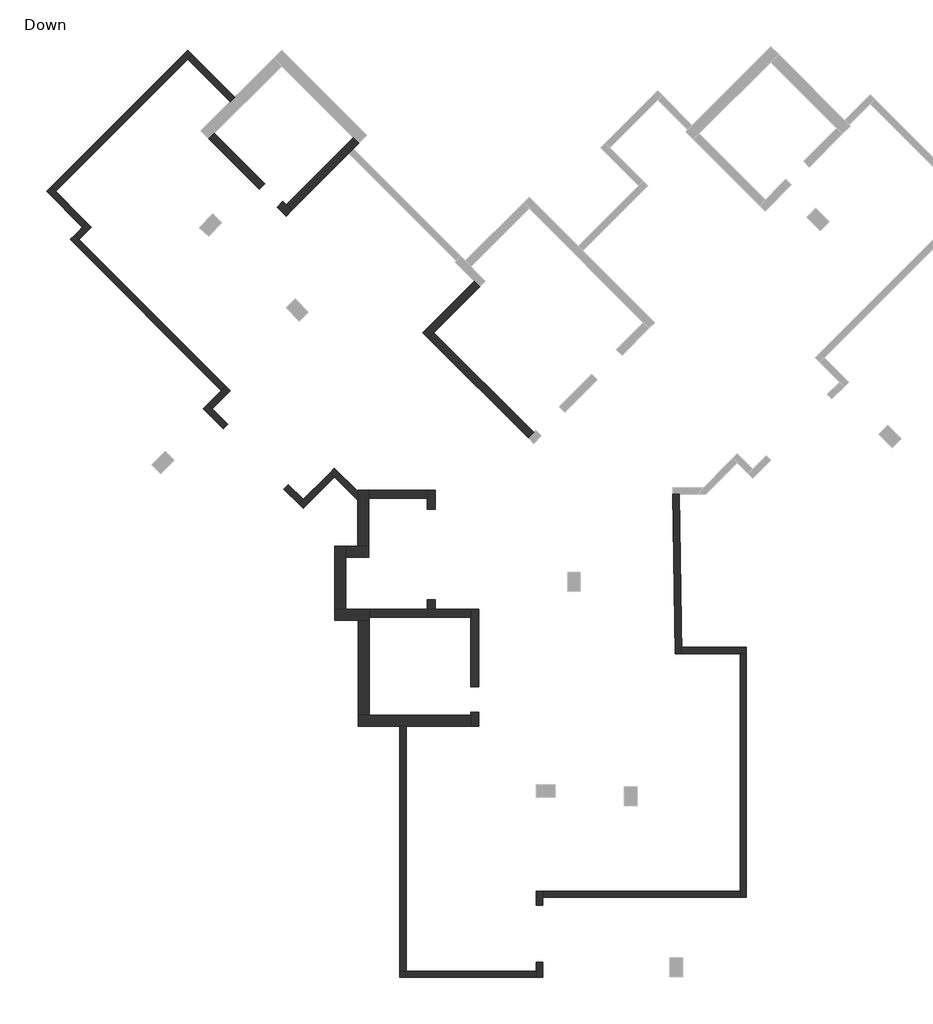
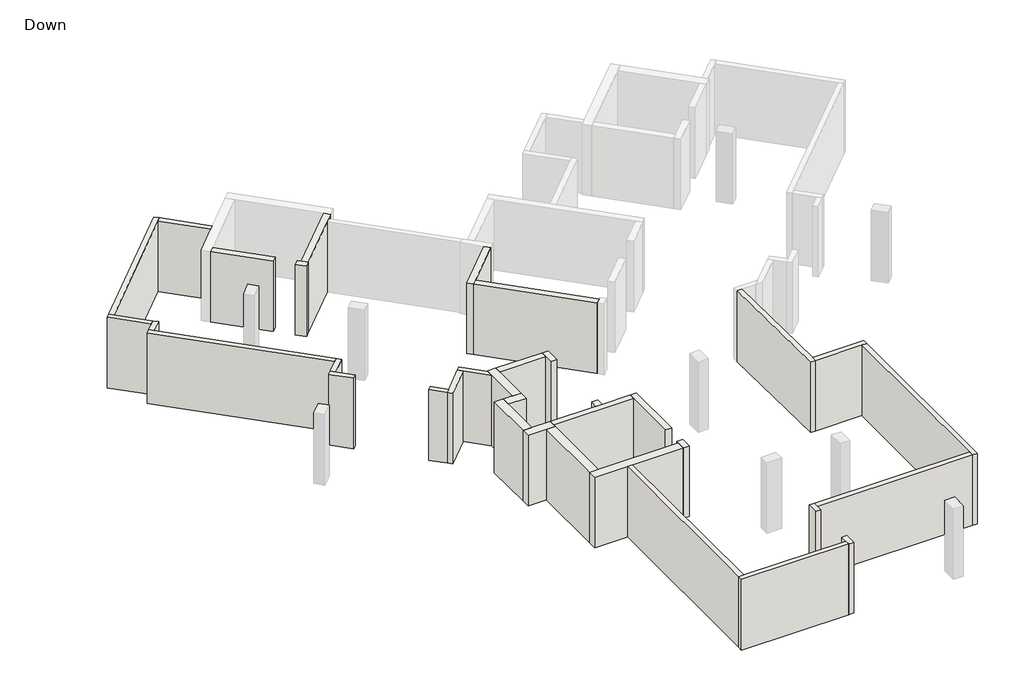
# One storey, part 1 of 2: 35 walls.
"""IFC4 building model written with IfcOpenShell, lengths in millimetres."""

import ifcopenshell
import ifcopenshell.guid

model = None  # the IFC model being written
_history = None  # IfcOwnerHistory: only IFC2X3 demands one
_inside = {}  # id of a spatial element -> (the spatial element, [elements in it])
_under = {}  # id of a project, library or spatial element -> (it, [spatial elements below it])
_declared = {}  # id of a project -> (the project, [libraries it declares])
_typed = {}  # id of a type object -> (the type object, [elements of that type])
_made_of = {}  # id of a material, layer set ... -> (it, [elements and type objects made of it])


def new_model(schema):
    """Start an empty IFC model of exactly this schema.

    Asked for "IFC4X3", IfcOpenShell would pick the latest addendum, in which some entities
    have other attributes; the version numbers below select the first issue.
    IFC2X3 requires an IfcOwnerHistory on every rooted entity: one is made here for all.
    """
    global model, _history
    if schema == "IFC4X3":
        model = ifcopenshell.file(schema_version=(4, 3, 0, 0))
    else:
        model = ifcopenshell.file(schema=schema)
    _inside.clear()
    _under.clear()
    _declared.clear()
    _typed.clear()
    _made_of.clear()
    _history = None
    if model.schema == "IFC2X3":
        org = make("IfcOrganization", Name="unknown")
        user = make(
            "IfcPersonAndOrganization",
            ThePerson=make("IfcPerson", FamilyName="unknown"),
            TheOrganization=org,
        )
        app = make(
            "IfcApplication",
            ApplicationDeveloper=org,
            Version="unknown",
            ApplicationFullName="unknown",
            ApplicationIdentifier="unknown",
        )
        _history = make(
            "IfcOwnerHistory",
            OwningUser=user,
            OwningApplication=app,
            ChangeAction="ADDED",
            CreationDate=0,
        )
    return model


def make(cls, **values):
    """One entity of the class cls with the attributes given. An attribute that is None is left unset."""
    return model.create_entity(
        cls, **{name: value for name, value in values.items() if value is not None}
    )


def rooted(cls, **values):
    """An entity with a GlobalId (a new one), such as an element, a storey or a relation."""
    return make(cls, GlobalId=ifcopenshell.guid.new(), OwnerHistory=_history, **values)


def si_unit(unit_type, name, prefix=None):
    """IfcSIUnit, for example si_unit("LENGTHUNIT", "METRE", prefix="MILLI")."""
    return make("IfcSIUnit", UnitType=unit_type, Prefix=prefix, Name=name)


def assignment(units):
    """IfcUnitAssignment: the units of a project."""
    return None if units is None else make("IfcUnitAssignment", Units=units)


def point(xyz):
    """IfcCartesianPoint."""
    return None if xyz is None else make("IfcCartesianPoint", Coordinates=xyz)


def direction(xyz):
    """IfcDirection."""
    return None if xyz is None else make("IfcDirection", DirectionRatios=xyz)


def frame(location, z_axis=None, x_axis=None):
    """IfcAxis2Placement3D, a coordinate frame: its origin and axes. An axis left out is left unset."""
    return make(
        "IfcAxis2Placement3D",
        Location=point(location),
        Axis=direction(z_axis),
        RefDirection=direction(x_axis),
    )


def origin():
    """The frame at (0, 0, 0) with its axes left unset."""
    return frame((0.0, 0.0, 0.0))


def origin_with_axes():
    """The frame at (0, 0, 0) with the z axis (0, 0, 1) and the x axis (1, 0, 0) written out."""
    return frame((0.0, 0.0, 0.0), z_axis=(0.0, 0.0, 1.0), x_axis=(1.0, 0.0, 0.0))


def place(relative_to, where):
    """IfcLocalPlacement: puts the frame where relative to a parent placement (None: the world)."""
    return make(
        "IfcLocalPlacement", PlacementRelTo=relative_to, RelativePlacement=where
    )


def context(
    kind, dimensions, precision=None, world=None, true_north=None, identifier=None
):
    """IfcGeometricRepresentationContext, for example the 3D "Model" context."""
    return make(
        "IfcGeometricRepresentationContext",
        ContextIdentifier=identifier,
        ContextType=kind,
        CoordinateSpaceDimension=dimensions,
        Precision=precision,
        WorldCoordinateSystem=world,
        TrueNorth=true_north,
    )


def project(units=None, contexts=None):
    """IfcProject with its units and contexts."""
    return rooted(
        "IfcProject",
        Name="project",
        RepresentationContexts=contexts,
        UnitsInContext=assignment(units),
    )


def spatial(cls, under=None, at=None, **own):
    """A site, building, storey or space (cls), placed at a placement, below another one or the project."""
    s = rooted(cls, ObjectPlacement=at, **own)
    if under is not None:
        _under.setdefault(under.id(), (under, []))[1].append(s)
    return s


def polyline(points):
    """IfcPolyline through the points."""
    return make("IfcPolyline", Points=[point(p) for p in points])


def outline(outer, holes=None, kind="AREA"):
    """IfcArbitraryClosedProfileDef: a profile drawn as a closed curve; with holes, ...WithVoids."""
    if holes is None:
        return make("IfcArbitraryClosedProfileDef", ProfileType=kind, OuterCurve=outer)
    return make(
        "IfcArbitraryProfileDefWithVoids",
        ProfileType=kind,
        OuterCurve=outer,
        InnerCurves=holes,
    )


def extrude(swept, where, along, depth):
    """IfcExtrudedAreaSolid: the profile swept, set in the frame where, extruded along a direction by depth."""
    return make(
        "IfcExtrudedAreaSolid",
        SweptArea=swept,
        Position=where,
        ExtrudedDirection=direction(along),
        Depth=depth,
    )


def faces_of(points, faces, orient=None, outer=None):
    """IfcFace entities. A face is a list of loops; a loop is a list of indices into points, from 0.

    orient and outer hold one flag for each loop. By default every Orientation is true, the
    first loop of a face is its IfcFaceOuterBound and the others are IfcFaceBound.
    """
    made = []
    for i, loops in enumerate(faces):
        bounds = []
        for j, loop in enumerate(loops):
            is_outer = j == 0 if outer is None else outer[i][j]
            bounds.append(
                make(
                    "IfcFaceOuterBound" if is_outer else "IfcFaceBound",
                    Bound=make("IfcPolyLoop", Polygon=[points[k] for k in loop]),
                    Orientation=True if orient is None else orient[i][j],
                )
            )
        made.append(make("IfcFace", Bounds=bounds))
    return made


def faceted_brep(points, faces, orient=None, outer=None, voids=None):
    """IfcFacetedBrep: a solid bounded by flat faces; with voids (closed shells), ...WithVoids."""
    shared = [point(p) for p in points]
    hull = make("IfcClosedShell", CfsFaces=faces_of(shared, faces, orient, outer))
    if voids is None:
        return make("IfcFacetedBrep", Outer=hull)
    return make(
        "IfcFacetedBrepWithVoids",
        Outer=hull,
        Voids=[
            make(cls, CfsFaces=faces_of(shared, fs, o, b)) for cls, fs, o, b in voids
        ],
    )


def shape(context_of_items, identifier, shape_type, items):
    """IfcShapeRepresentation: the items that make up one representation, for example the "Body"."""
    return make(
        "IfcShapeRepresentation",
        ContextOfItems=context_of_items,
        RepresentationIdentifier=identifier,
        RepresentationType=shape_type,
        Items=items,
    )


def made_of(thing, what):
    """Note that an element or type object is made of a material, layer set ...; save() writes the relation."""
    if what is not None:
        _made_of.setdefault(what.id(), (what, []))[1].append(thing)
    return thing


def element(
    cls,
    number,
    at=None,
    inside=None,
    cuts=None,
    type_object=None,
    material=None,
    context=None,
    identifier="Body",
    shape_type=None,
    held_by="IfcProductDefinitionShape",
    body=None,
    shapes=None,
    **own,
):
    """One element of the class cls, such as IfcWall. Its Tag is "e" and its number.

    at: its placement. inside: the storey or other place that contains it. cuts: it is an
    opening in that element (IfcRelVoidsElement). A single representation is given by context,
    identifier, shape_type and body (its items); several are given by shapes. held_by: the class
    of the entity that holds the representations. save() writes the other relations.
    """
    e = rooted(cls, Tag="e%d" % number, ObjectPlacement=at, **own)
    if body is not None:
        shapes = [shape(context, identifier, shape_type, body)]
    if shapes is not None:
        e.Representation = make(held_by, Representations=shapes)
    if inside is not None:
        _inside.setdefault(inside.id(), (inside, []))[1].append(e)
    if cuts is not None:
        rooted(
            "IfcRelVoidsElement", RelatingBuildingElement=cuts, RelatedOpeningElement=e
        )
    if type_object is not None:
        _typed.setdefault(type_object.id(), (type_object, []))[1].append(e)
    return made_of(e, material)


def aggregate(whole, parts):
    """IfcRelAggregates: a whole, such as a stair, and the parts it consists of."""
    return rooted("IfcRelAggregates", RelatingObject=whole, RelatedObjects=parts)


def save(model, path):
    """Write the relations noted so far, then the file.

    IfcRelAggregates (storeys below a building ...), IfcRelContainedInSpatialStructure (elements
    in a storey), IfcRelDefinesByType, IfcRelAssociatesMaterial and IfcRelDeclares: one each for
    every whole, place, type object, material and project.
    """
    for whole, parts in _under.values():
        aggregate(whole, parts)
    for where, things in _inside.values():
        rooted(
            "IfcRelContainedInSpatialStructure",
            RelatedElements=things,
            RelatingStructure=where,
        )
    for kind, things in _typed.values():
        rooted("IfcRelDefinesByType", RelatedObjects=things, RelatingType=kind)
    for what, things in _made_of.values():
        rooted("IfcRelAssociatesMaterial", RelatedObjects=things, RelatingMaterial=what)
    for by, libraries in _declared.values():
        rooted("IfcRelDeclares", RelatingContext=by, RelatedDefinitions=libraries)
    model.write(path)


model = new_model("IFC4")

# Units and contexts
model_context = context("Model", 3, world=origin())
ifc_project = project(units=[si_unit("LENGTHUNIT", "METRE", prefix="MILLI")], contexts=[model_context])

# Site, building, storey
site = spatial("IfcSite", under=ifc_project)
building = spatial("IfcBuilding", under=site)
storey = spatial("IfcBuildingStorey", under=building, Name="Down", Elevation=0.0)

# Walls
placement = place(None, origin())
element("IfcWall", 1, ObjectType="20", at=placement, inside=storey, context=model_context, shape_type="Brep", body=[
    faceted_brep([(-4151.5371537, 1666.662681, 0.0), (-4879.6277554, 2394.7532827, 0.0), (-4879.6277554, 2394.7532827, 2820.0), (-4879.6277554, 2394.7532827, 3000.0), (-4151.5371537, 1666.662681, 3000.0), (-4151.5371537, 1666.662681, 2820.0), (-4151.5371537, 1383.8199686, 0.0), (-4151.5371537, 1383.8199686, 3000.0), (-4879.6277554, 2111.9105702, 3000.0), (-5021.0491116, 2253.3319265, 3000.0), (-5021.0491116, 2253.3319265, 0.0), (-4879.6277554, 2111.9105702, 0.0)], [[[0, 1, 2, 3, 4, 5]], [[6, 7, 8, 9, 10, 11]], [[1, 0, 6, 11, 10]], [[4, 3, 9, 8, 7]], [[3, 2, 1, 10, 9]], [[0, 5, 4, 7, 6]]]),
])
element("IfcWall", 2, ObjectType="20", at=placement, inside=storey, context=model_context, shape_type="Brep", body=[
    faceted_brep([(-5021.0491116, 2253.3319265, 0.0), (-5869.5772491, 1404.803789, 0.0), (-6010.9986053, 1263.3824328, 0.0), (-6010.9986053, 1263.3824328, 3000.0), (-5869.5772491, 1404.803789, 3000.0), (-5021.0491116, 2253.3319265, 3000.0), (-4879.6277554, 2111.9105702, 0.0), (-4879.6277554, 2111.9105702, 3000.0), (-5869.5772491, 1121.9610766, 3000.0), (-5869.5772491, 1121.9610766, 0.0), (-5945.8975357, 1198.2813632, 3000.0)], [[[0, 1, 2, 3, 4, 5]], [[6, 7, 8, 9]], [[2, 1, 0, 6, 9]], [[5, 4, 3, 10, 8, 7]], [[0, 5, 7, 6]], [[3, 2, 9, 8, 10]]]),
])
element("IfcWall", 3, ObjectType="20", at=placement, inside=storey, context=model_context, shape_type="Brep", body=[
    faceted_brep([(-5869.5772491, 1404.803789, 0.0), (-6335.1870225, 1870.4135624, 0.0), (-6335.1870225, 1870.4135624, 2820.0), (-6335.1870225, 1870.4135624, 3000.0), (-5869.5772491, 1404.803789, 3000.0), (-5869.5772491, 1404.803789, 2820.0), (-6010.9986053, 1263.3824328, 0.0), (-6010.9986053, 1263.3824328, 3000.0), (-6476.6083787, 1728.9922062, 3000.0), (-6476.6083787, 1728.9922062, 2820.0), (-6476.6083787, 1728.9922062, 0.0)], [[[0, 1, 2, 3, 4, 5]], [[6, 7, 8, 9, 10]], [[1, 0, 6, 10]], [[3, 2, 1, 10, 9, 8]], [[4, 3, 8, 7]], [[0, 5, 4, 7, 6]]]),
])
element("IfcWall", 4, ObjectType="20", at=placement, inside=storey, context=model_context, shape_type="Brep", body=[
    faceted_brep([(-8243.933641, 3779.160181, 0.0), (-8738.7611577, 4273.9876976, 0.0), (-8880.1825139, 4415.4090539, 0.0), (-8880.1825139, 4415.4090539, 3000.0), (-8738.7611577, 4273.9876976, 3000.0), (-8243.933641, 3779.160181, 3000.0), (-8243.933641, 3779.160181, 2820.0), (-8385.3549973, 3637.7388248, 0.0), (-8385.3549973, 3637.7388248, 2820.0), (-8385.3549973, 3637.7388248, 3000.0), (-8946.5252944, 4198.9091219, 3000.0), (-9021.6038701, 4273.9876976, 3000.0), (-9021.6038701, 4273.9876976, 0.0)], [[[0, 1, 2, 3, 4, 5, 6]], [[7, 8, 9, 10, 11, 12]], [[2, 1, 0, 7, 12]], [[5, 4, 3, 11, 10, 9]], [[0, 6, 5, 9, 8, 7]], [[3, 2, 12, 11]]]),
])
element("IfcWall", 5, ObjectType="20", at=placement, inside=storey, context=model_context, shape_type="Brep", body=[
    faceted_brep([(-8738.7611577, 4273.9876976, 0.0), (-8172.2562086, 4840.4926467, 0.0), (-8172.2562086, 4840.4926467, 2820.0), (-8172.2562086, 4840.4926467, 3000.0), (-8738.7611577, 4273.9876976, 3000.0), (-8738.7611577, 4273.9876976, 2820.0), (-8880.1825139, 4415.4090539, 0.0), (-8880.1825139, 4415.4090539, 3000.0), (-8455.0989211, 4840.4926467, 3000.0), (-8313.6775649, 4981.9140029, 3000.0), (-8313.6775649, 4981.9140029, 0.0), (-8455.0989211, 4840.4926467, 0.0)], [[[0, 1, 2, 3, 4, 5]], [[6, 7, 8, 9, 10, 11]], [[1, 0, 6, 11, 10]], [[4, 3, 9, 8, 7]], [[0, 5, 4, 7, 6]], [[3, 2, 1, 10, 9]]]),
])
element("IfcWall", 6, ObjectType="20", at=placement, inside=storey, context=model_context, shape_type="Brep", body=[
    faceted_brep([(-8313.6775649, 4981.9140029, 0.0), (-12945.5654963, 9613.8019343, 0.0), (-13086.9868525, 9755.2232905, 0.0), (-13086.9868525, 9755.2232905, 3000.0), (-12945.5654963, 9613.8019343, 3000.0), (-8313.6775649, 4981.9140029, 3000.0), (-13228.4082088, 9613.8019343, 0.0), (-8455.0989211, 4840.4926467, 0.0), (-8455.0989211, 4840.4926467, 3000.0), (-13228.4082088, 9613.8019343, 3000.0)], [[[0, 1, 2, 3, 4, 5]], [[6, 7, 8, 9]], [[2, 1, 0, 7, 6]], [[5, 4, 3, 9, 8]], [[3, 2, 6, 9]], [[0, 5, 8, 7]]]),
])
element("IfcWall", 7, ObjectType="20", at=placement, inside=storey, context=model_context, shape_type="Brep", body=[
    faceted_brep([(-12945.5654963, 9613.8019343, 0.0), (-12556.7794585, 10002.5879721, 0.0), (-12556.7794585, 10002.5879721, 2820.0), (-12556.7794585, 10002.5879721, 3000.0), (-12945.5654963, 9613.8019343, 3000.0), (-12945.5654963, 9613.8019343, 2820.0), (-13086.9868525, 9755.2232905, 0.0), (-13086.9868525, 9755.2232905, 3000.0), (-12839.6221709, 10002.5879721, 3000.0), (-12698.2008147, 10144.0093284, 3000.0), (-12698.2008147, 10144.0093284, 0.0), (-12839.6221709, 10002.5879721, 0.0)], [[[0, 1, 2, 3, 4, 5]], [[6, 7, 8, 9, 10, 11]], [[1, 0, 6, 11, 10]], [[4, 3, 9, 8, 7]], [[0, 5, 4, 7, 6]], [[3, 2, 1, 10, 9]]]),
])
element("IfcWall", 8, ObjectType="20", at=placement, inside=storey, context=model_context, shape_type="Brep", body=[
    faceted_brep([(-12698.2008147, 10144.0093284, 0.0), (-13688.6426542, 11134.4511678, 0.0), (-13830.0640104, 11275.8725241, 0.0), (-13830.0640104, 11275.8725241, 3000.0), (-13688.6426542, 11134.4511678, 3000.0), (-12698.2008147, 10144.0093284, 3000.0), (-12839.6221709, 10002.5879721, 0.0), (-12839.6221709, 10002.5879721, 3000.0), (-13971.4853667, 11134.4511678, 3000.0), (-13971.4853667, 11134.4511678, 0.0)], [[[0, 1, 2, 3, 4, 5]], [[6, 7, 8, 9]], [[2, 1, 0, 6, 9]], [[5, 4, 3, 8, 7]], [[0, 5, 7, 6]], [[3, 2, 9, 8]]]),
])
element("IfcWall", 9, ObjectType="20", at=placement, inside=storey, context=model_context, shape_type="Brep", body=[
    faceted_brep([(-13688.6426542, 11134.4511678, 0.0), (-9516.9564504, 15306.1373716, 0.0), (-9375.5350942, 15447.5587279, 0.0), (-9375.5350942, 15447.5587279, 3000.0), (-9516.9564504, 15306.1373716, 3000.0), (-13688.6426542, 11134.4511678, 3000.0), (-13688.6426542, 11134.4511678, 2820.0), (-13830.0640104, 11275.8725241, 0.0), (-13830.0640104, 11275.8725241, 3000.0), (-9516.9564504, 15588.9800841, 3000.0), (-9516.9564504, 15588.9800841, 0.0)], [[[0, 1, 2, 3, 4, 5, 6]], [[7, 8, 9, 10]], [[2, 1, 0, 7, 10]], [[5, 4, 3, 9, 8]], [[0, 6, 5, 8, 7]], [[3, 2, 10, 9]]]),
])
element("IfcWall", 10, ObjectType="20", at=placement, inside=storey, context=model_context, shape_type="Brep", body=[
    faceted_brep([(-9516.9564504, 15306.1373716, 0.0), (-8173.4037002, 13962.5846214, 0.0), (-8173.4037002, 13962.5846214, 2820.0), (-8173.4037002, 13962.5846214, 3000.0), (-9516.9564504, 15306.1373716, 3000.0), (-9516.9564504, 15306.1373716, 2820.0), (-9375.5350942, 15447.5587279, 0.0), (-9375.5350942, 15447.5587279, 3000.0), (-8031.9823439, 14104.0059776, 3000.0), (-8031.9823439, 14104.0059776, 0.0)], [[[0, 1, 2, 3, 4, 5]], [[6, 7, 8, 9]], [[1, 0, 6, 9]], [[4, 3, 8, 7]], [[0, 5, 4, 7, 6]], [[3, 2, 1, 9, 8]]]),
])
element("IfcWall", 11, ObjectType="20", at=placement, inside=storey, context=model_context, shape_type="Brep", body=[
    faceted_brep([(5808.4890075, 1568.8966142, 0.0), (5879.1909347, -3458.8761541, 0.0), (5879.1909347, -3458.8761541, 2820.0), (5879.1909347, -3458.8761541, 3000.0), (5808.4890075, 1568.8966142, 3000.0), (6008.5087812, 1568.8966142, 0.0), (6008.5087812, 1568.8966142, 3000.0), (6076.3982534, -3258.8761541, 3000.0), (6079.2107085, -3458.8761541, 3000.0), (6079.2107085, -3458.8761541, 0.0), (6076.3982534, -3258.8761541, 0.0)], [[[0, 1, 2, 3, 4]], [[5, 6, 7, 8, 9, 10]], [[1, 0, 5, 10, 9]], [[4, 3, 8, 7, 6]], [[0, 4, 6, 5]], [[3, 2, 1, 9, 8]]]),
])
element("IfcWall", 12, ObjectType="20", at=placement, inside=storey, context=model_context, shape_type="Brep", body=[
    faceted_brep([(6079.2107085, -3458.8761541, 0.0), (7926.5061285, -3458.8761541, 0.0), (8126.5061285, -3458.8761541, 0.0), (8126.5061285, -3458.8761541, 3000.0), (7926.5061285, -3458.8761541, 3000.0), (6079.2107085, -3458.8761541, 3000.0), (6076.3982534, -3258.8761541, 0.0), (6076.3982534, -3258.8761541, 3000.0), (8126.5061285, -3258.8761541, 3000.0), (8126.5061285, -3258.8761541, 0.0)], [[[0, 1, 2, 3, 4, 5]], [[6, 7, 8, 9]], [[2, 1, 0, 6, 9]], [[5, 4, 3, 8, 7]], [[0, 5, 7, 6]], [[3, 2, 9, 8]]]),
])
element("IfcWall", 13, ObjectType="20", at=placement, inside=storey, context=model_context, shape_type="Brep", body=[
    faceted_brep([(7926.5061285, -3458.8761541, 0.0), (7926.5061285, -10958.0646121, 0.0), (7926.5061285, -11158.0646121, 0.0), (7926.5061285, -11158.0646121, 3000.0), (7926.5061285, -10958.0646121, 3000.0), (7926.5061285, -3458.8761541, 3000.0), (7926.5061285, -3458.8761541, 2820.0), (8126.5061285, -3458.8761541, 0.0), (8126.5061285, -3458.8761541, 3000.0), (8126.5061285, -11158.0646121, 3000.0), (8126.5061285, -11158.0646121, 0.0)], [[[0, 1, 2, 3, 4, 5, 6]], [[7, 8, 9, 10]], [[2, 1, 0, 7, 10]], [[5, 4, 3, 9, 8]], [[0, 6, 5, 8, 7]], [[3, 2, 10, 9]]]),
])
element("IfcWall", 14, ObjectType="20", at=placement, inside=storey, context=model_context, shape_type="Brep", body=[
    faceted_brep([(7926.5061285, -10958.0646121, 0.0), (1689.535885, -10958.0646121, 0.0), (1689.535885, -10958.0646121, 3000.0), (7926.5061285, -10958.0646121, 3000.0), (7926.5061285, -10958.0646121, 2820.0), (7926.5061285, -11158.0646121, 0.0), (7926.5061285, -11158.0646121, 3000.0), (6112.9804297, -11158.0646121, 3000.0), (1689.535885, -11158.0646121, 3000.0), (1689.535885, -11158.0646121, 2820.0), (1689.535885, -11158.0646121, 0.0)], [[[0, 1, 2, 3, 4]], [[5, 6, 7, 8, 9, 10]], [[1, 0, 5, 10]], [[3, 2, 8, 7, 6]], [[0, 4, 3, 6, 5]], [[2, 1, 10, 9, 8]]]),
])
element("IfcWall", 15, ObjectType="20", at=placement, inside=storey, context=model_context, shape_type="Brep", body=[
    faceted_brep([(1489.535885, -10958.0646121, 0.0), (1489.535885, -11409.1015824, 0.0), (1489.535885, -11409.1015824, 2820.0), (1489.535885, -11409.1015824, 3000.0), (1489.535885, -10958.0646121, 3000.0), (1489.535885, -10958.0646121, 2820.0), (1689.535885, -10958.0646121, 0.0), (1689.535885, -10958.0646121, 3000.0), (1689.535885, -11158.0646121, 3000.0), (1689.535885, -11409.1015824, 3000.0), (1689.535885, -11409.1015824, 2820.0), (1689.535885, -11409.1015824, 0.0), (1689.535885, -11158.0646121, 0.0)], [[[0, 1, 2, 3, 4, 5]], [[6, 7, 8, 9, 10, 11, 12]], [[1, 0, 6, 12, 11]], [[3, 2, 1, 11, 10, 9]], [[4, 3, 9, 8, 7]], [[0, 5, 4, 7, 6]]]),
])
element("IfcWall", 16, ObjectType="20", at=placement, inside=storey, context=model_context, shape_type="Brep", body=[
    faceted_brep([(1489.535885, -13208.1998691, 0.0), (1489.535885, -13487.1899503, 0.0), (1489.535885, -13687.1899503, 0.0), (1489.535885, -13687.1899503, 3000.0), (1489.535885, -13487.1899503, 3000.0), (1489.535885, -13208.1998691, 3000.0), (1489.535885, -13208.1998691, 2820.0), (1689.535885, -13208.1998691, 0.0), (1689.535885, -13208.1998691, 2820.0), (1689.535885, -13208.1998691, 3000.0), (1689.535885, -13687.1899503, 3000.0), (1689.535885, -13687.1899503, 2820.0), (1689.535885, -13687.1899503, 0.0), (1589.2653711, -13687.1899503, 3000.0)], [[[0, 1, 2, 3, 4, 5, 6]], [[7, 8, 9, 10, 11, 12]], [[2, 1, 0, 7, 12]], [[5, 4, 3, 13, 10, 9]], [[0, 6, 5, 9, 8, 7]], [[3, 2, 12, 11, 10, 13]]]),
])
element("IfcWall", 17, ObjectType="20", at=placement, inside=storey, context=model_context, shape_type="Brep", body=[
    faceted_brep([(1489.535885, -13487.1899503, 0.0), (-2615.4235379, -13487.1899503, 0.0), (-2815.4235379, -13487.1899503, 0.0), (-2815.4235379, -13487.1899503, 3000.0), (-2615.4235379, -13487.1899503, 3000.0), (1489.535885, -13487.1899503, 3000.0), (1489.535885, -13487.1899503, 2820.0), (1489.535885, -13687.1899503, 0.0), (1489.535885, -13687.1899503, 3000.0), (-2815.4235379, -13687.1899503, 3000.0), (-2815.4235379, -13687.1899503, 0.0)], [[[0, 1, 2, 3, 4, 5, 6]], [[7, 8, 9, 10]], [[2, 1, 0, 7, 10]], [[5, 4, 3, 9, 8]], [[0, 6, 5, 8, 7]], [[3, 2, 10, 9]]]),
])
element("IfcWall", 18, ObjectType="20", at=placement, inside=storey, context=model_context, shape_type="Brep", body=[
    faceted_brep([(-2615.4235379, -13487.1899503, 0.0), (-2615.4235379, -5759.3270107, 0.0), (-2615.4235379, -5759.3270107, 2820.0), (-2615.4235379, -5759.3270107, 3000.0), (-2615.4235379, -13487.1899503, 3000.0), (-2615.4235379, -13487.1899503, 2820.0), (-2815.4235379, -13487.1899503, 0.0), (-2815.4235379, -13487.1899503, 3000.0), (-2815.4235379, -5759.3270107, 3000.0), (-2815.4235379, -5759.3270107, 0.0)], [[[0, 1, 2, 3, 4, 5]], [[6, 7, 8, 9]], [[1, 0, 6, 9]], [[4, 3, 8, 7]], [[0, 5, 4, 7, 6]], [[3, 2, 1, 9, 8]]]),
])
element("IfcWall", 19, ObjectType="25", at=placement, inside=storey, context=model_context, shape_type="Brep", body=[
    faceted_brep([(-8848.1886442, 12792.8249306, 0.0), (-7257.2630329, 11201.8993193, 0.0), (-7257.2630329, 11201.8993193, 2820.0), (-7257.2630329, 11201.8993193, 3000.0), (-8848.1886442, 12792.8249306, 3000.0), (-8671.4119489, 12969.6016259, 0.0), (-8671.4119489, 12969.6016259, 2820.0), (-8671.4119489, 12969.6016259, 3000.0), (-7080.4863376, 11378.6760146, 3000.0), (-7080.4863376, 11378.6760146, 2820.0), (-7080.4863376, 11378.6760146, 0.0)], [[[0, 1, 2, 3, 4]], [[5, 6, 7, 8, 9, 10]], [[1, 0, 5, 10]], [[3, 2, 1, 10, 9, 8]], [[4, 3, 8, 7]], [[0, 4, 7, 6, 5]]]),
])
element("IfcWall", 20, ObjectType="25", at=placement, inside=storey, context=model_context, shape_type="Brep", body=[
    faceted_brep([(-6231.7938218, 10529.9834989, 0.0), (-6408.5705171, 10706.7601941, 0.0), (-6515.2924693, 10813.4821463, 0.0), (-6515.2924693, 10813.4821463, 2820.0), (-6515.2924693, 10813.4821463, 3000.0), (-6408.5705171, 10706.7601941, 3000.0), (-6231.7938218, 10529.9834989, 3000.0), (-6408.5705171, 10353.2068036, 0.0), (-6408.5705171, 10353.2068036, 2820.0), (-6408.5705171, 10353.2068036, 3000.0), (-6692.0691646, 10636.705451, 3000.0), (-6692.0691646, 10636.705451, 2820.0), (-6692.0691646, 10636.705451, 0.0)], [[[0, 1, 2, 3, 4, 5, 6]], [[7, 8, 9, 10, 11, 12]], [[2, 1, 0, 7, 12]], [[4, 3, 2, 12, 11, 10]], [[6, 5, 4, 10, 9]], [[0, 6, 9, 8, 7]]]),
])
element("IfcWall", 21, ObjectType="25", at=placement, inside=storey, context=model_context, shape_type="Brep", body=[
    faceted_brep([(-6231.7938218, 10529.9834989, 0.0), (-4429.582499, 12332.1948217, 0.0), (-4288.1611428, 12473.6161779, 0.0), (-4110.3410285, 12651.4362922, 0.0), (-4110.3410285, 12651.4362922, 3000.0), (-4288.1611428, 12473.6161779, 3000.0), (-4429.582499, 12332.1948217, 3000.0), (-6231.7938218, 10529.9834989, 3000.0), (-6408.5705171, 10706.7601941, 0.0), (-6408.5705171, 10706.7601941, 2820.0), (-6408.5705171, 10706.7601941, 3000.0), (-4287.1177238, 12828.2129875, 3000.0), (-4287.1177238, 12828.2129875, 2820.0), (-4287.1177238, 12828.2129875, 0.0)], [[[0, 1, 2, 3, 4, 5, 6, 7]], [[8, 9, 10, 11, 12, 13]], [[3, 2, 1, 0, 8, 13]], [[7, 6, 5, 4, 11, 10]], [[4, 3, 13, 12, 11]], [[0, 7, 10, 9, 8]]]),
])
element("IfcWall", 22, ObjectType="25", at=placement, inside=storey, context=model_context, shape_type="Brep", body=[
    faceted_brep([(-468.8867571, 8300.9074348, 0.0), (-2095.1940493, 6674.6001426, 0.0), (-2095.1940493, 6674.6001426, 2820.0), (-2095.1940493, 6674.6001426, 3000.0), (-468.8867571, 8300.9074348, 3000.0), (-468.8867571, 8300.9074348, 2820.0), (-292.1100618, 8124.1307395, 0.0), (-292.1100618, 8124.1307395, 3000.0), (-1741.6406587, 6674.6001426, 3000.0), (-1918.417354, 6497.8234473, 3000.0), (-1918.417354, 6497.8234473, 0.0), (-1741.6406587, 6674.6001426, 0.0)], [[[0, 1, 2, 3, 4, 5]], [[6, 7, 8, 9, 10, 11]], [[1, 0, 6, 11, 10]], [[4, 3, 9, 8, 7]], [[0, 5, 4, 7, 6]], [[3, 2, 1, 10, 9]]]),
])
element("IfcWall", 23, ObjectType="25", at=placement, inside=storey, context=model_context, shape_type="SweptSolid", body=[
    extrude(outline(polyline([(1231.0458064, 3348.3602869), (-1918.417354, 6497.8234473), (-1741.6406587, 6674.6001426), (1407.8225017, 3525.1369821), (1231.0458064, 3348.3602869)])), origin_with_axes(), (0.0, 0.0, 1.0), 3000.0),
])
element("IfcWall", 24, ObjectType="25", at=placement, inside=storey, context=model_context, shape_type="Brep", body=[
    faceted_brep([(-326.6949536, -5759.3270107, 0.0), (-326.6949536, -5309.9131243, 0.0), (-326.6949536, -5309.9131243, 2820.0), (-326.6949536, -5309.9131243, 3000.0), (-326.6949536, -5759.3270107, 3000.0), (-326.6949536, -5759.3270107, 2820.0), (-576.6949536, -5759.3270107, 0.0), (-576.6949536, -5759.3270107, 3000.0), (-576.6949536, -5409.3270107, 3000.0), (-576.6949536, -5309.9131243, 3000.0), (-576.6949536, -5309.9131243, 2820.0), (-576.6949536, -5309.9131243, 0.0), (-576.6949536, -5409.3270107, 0.0)], [[[0, 1, 2, 3, 4, 5]], [[6, 7, 8, 9, 10, 11, 12]], [[1, 0, 6, 12, 11]], [[3, 2, 1, 11, 10, 9]], [[4, 3, 9, 8, 7]], [[0, 5, 4, 7, 6]]]),
])
element("IfcWall", 25, ObjectType="25", at=placement, inside=storey, context=model_context, shape_type="Brep", body=[
    faceted_brep([(-326.6949536, -4509.9131243, 0.0), (-326.6949536, -2059.417182, 0.0), (-326.6949536, -2059.417182, 2820.0), (-326.6949536, -2059.417182, 3000.0), (-326.6949536, -4509.9131243, 3000.0), (-326.6949536, -4509.9131243, 2820.0), (-576.6949536, -4509.9131243, 0.0), (-576.6949536, -4509.9131243, 2820.0), (-576.6949536, -4509.9131243, 3000.0), (-576.6949536, -2309.417182, 3000.0), (-576.6949536, -2059.417182, 3000.0), (-576.6949536, -2059.417182, 0.0), (-576.6949536, -2309.417182, 0.0)], [[[0, 1, 2, 3, 4, 5]], [[6, 7, 8, 9, 10, 11, 12]], [[1, 0, 6, 12, 11]], [[4, 3, 10, 9, 8]], [[0, 5, 4, 8, 7, 6]], [[3, 2, 1, 11, 10]]]),
])
element("IfcWall", 26, ObjectType="25", at=placement, inside=storey, context=model_context, shape_type="Brep", body=[
    faceted_brep([(-576.6949536, -2059.417182, 0.0), (-1697.2991014, -2059.417182, 0.0), (-1947.2991014, -2059.417182, 0.0), (-3786.2531141, -2059.417182, 0.0), (-3786.2531141, -2059.417182, 3000.0), (-1947.2991014, -2059.417182, 3000.0), (-1697.2991014, -2059.417182, 3000.0), (-576.6949536, -2059.417182, 3000.0), (-576.6949536, -2309.417182, 0.0), (-576.6949536, -2309.417182, 2820.0), (-576.6949536, -2309.417182, 3000.0), (-3786.2531141, -2309.417182, 3000.0), (-3786.2531141, -2309.417182, 2820.0), (-3786.2531141, -2309.417182, 0.0)], [[[0, 1, 2, 3, 4, 5, 6, 7]], [[8, 9, 10, 11, 12, 13]], [[3, 2, 1, 0, 8, 13]], [[7, 6, 5, 4, 11, 10]], [[0, 7, 10, 9, 8]], [[4, 3, 13, 12, 11]]]),
])
element("IfcWall", 27, ObjectType="25", at=placement, inside=storey, context=model_context, shape_type="Brep", body=[
    faceted_brep([(-1697.2991014, -2059.417182, 0.0), (-1697.2991014, -1759.417182, 0.0), (-1697.2991014, -1759.417182, 2820.0), (-1697.2991014, -1759.417182, 3000.0), (-1697.2991014, -2059.417182, 3000.0), (-1697.2991014, -2059.417182, 2820.0), (-1947.2991014, -2059.417182, 0.0), (-1947.2991014, -2059.417182, 3000.0), (-1947.2991014, -1759.417182, 3000.0), (-1947.2991014, -1759.417182, 2820.0), (-1947.2991014, -1759.417182, 0.0)], [[[0, 1, 2, 3, 4, 5]], [[6, 7, 8, 9, 10]], [[1, 0, 6, 10]], [[3, 2, 1, 10, 9, 8]], [[4, 3, 8, 7]], [[0, 5, 4, 7, 6]]]),
])
element("IfcWall", 28, ObjectType="25", at=placement, inside=storey, context=model_context, shape_type="Brep", body=[
    faceted_brep([(-1697.2991014, 1090.0868757, 0.0), (-1697.2991014, 1690.0868757, 0.0), (-1697.2991014, 1690.0868757, 2820.0), (-1697.2991014, 1690.0868757, 3000.0), (-1697.2991014, 1090.0868757, 3000.0), (-1697.2991014, 1090.0868757, 2820.0), (-1947.2991014, 1090.0868757, 0.0), (-1947.2991014, 1090.0868757, 2820.0), (-1947.2991014, 1090.0868757, 3000.0), (-1947.2991014, 1440.0868757, 3000.0), (-1947.2991014, 1690.0868757, 3000.0), (-1947.2991014, 1690.0868757, 0.0), (-1947.2991014, 1440.0868757, 0.0)], [[[0, 1, 2, 3, 4, 5]], [[6, 7, 8, 9, 10, 11, 12]], [[1, 0, 6, 12, 11]], [[4, 3, 10, 9, 8]], [[0, 5, 4, 8, 7, 6]], [[3, 2, 1, 11, 10]]]),
])
element("IfcWall", 29, ObjectType="25", at=placement, inside=storey, context=model_context, shape_type="Brep", body=[
    faceted_brep([(-1947.2991014, 1690.0868757, 0.0), (-3801.5371537, 1690.0868757, 0.0), (-3801.5371537, 1690.0868757, 2820.0), (-3801.5371537, 1690.0868757, 3000.0), (-1947.2991014, 1690.0868757, 3000.0), (-1947.2991014, 1440.0868757, 0.0), (-1947.2991014, 1440.0868757, 3000.0), (-3801.5371537, 1440.0868757, 3000.0), (-3801.5371537, 1440.0868757, 0.0)], [[[0, 1, 2, 3, 4]], [[5, 6, 7, 8]], [[1, 0, 5, 8]], [[4, 3, 7, 6]], [[0, 4, 6, 5]], [[3, 2, 1, 8, 7]]]),
])
element("IfcWall", 30, ObjectType="35", at=placement, inside=storey, context=model_context, shape_type="Brep", body=[
    faceted_brep([(-576.6949536, -5409.3270107, 0.0), (-3786.2531141, -5409.3270107, 0.0), (-4136.2531141, -5409.3270107, 0.0), (-4136.2531141, -5409.3270107, 3000.0), (-3786.2531141, -5409.3270107, 3000.0), (-576.6949536, -5409.3270107, 3000.0), (-576.6949536, -5409.3270107, 2820.0), (-576.6949536, -5759.3270107, 0.0), (-576.6949536, -5759.3270107, 3000.0), (-2615.4235379, -5759.3270107, 3000.0), (-2815.4235379, -5759.3270107, 3000.0), (-4136.2531141, -5759.3270107, 3000.0), (-4136.2531141, -5759.3270107, 0.0), (-2815.4235379, -5759.3270107, 0.0), (-2615.4235379, -5759.3270107, 0.0)], [[[0, 1, 2, 3, 4, 5, 6]], [[7, 8, 9, 10, 11, 12, 13, 14]], [[2, 1, 0, 7, 14, 13, 12]], [[5, 4, 3, 11, 10, 9, 8]], [[3, 2, 12, 11]], [[0, 6, 5, 8, 7]]]),
])
element("IfcWall", 31, ObjectType="35", at=placement, inside=storey, context=model_context, shape_type="Brep", body=[
    faceted_brep([(-3786.2531141, -5409.3270107, 0.0), (-3786.2531141, -2409.417182, 0.0), (-3786.2531141, -2409.417182, 3000.0), (-3786.2531141, -5409.3270107, 3000.0), (-3786.2531141, -5409.3270107, 2820.0), (-4136.2531141, -5409.3270107, 0.0), (-4136.2531141, -5409.3270107, 3000.0), (-4136.2531141, -2409.417182, 3000.0), (-4136.2531141, -2409.417182, 0.0)], [[[0, 1, 2, 3, 4]], [[5, 6, 7, 8]], [[1, 0, 5, 8]], [[3, 2, 7, 6]], [[0, 4, 3, 6, 5]], [[2, 1, 8, 7]]]),
])
element("IfcWall", 32, ObjectType="35", at=placement, inside=storey, context=model_context, shape_type="Brep", body=[
    faceted_brep([(-3786.2531141, -2059.417182, 0.0), (-4525.1449692, -2059.417182, 0.0), (-4875.1449692, -2059.417182, 0.0), (-4875.1449692, -2059.417182, 3000.0), (-4525.1449692, -2059.417182, 3000.0), (-3786.2531141, -2059.417182, 3000.0), (-3786.2531141, -2409.417182, 0.0), (-3786.2531141, -2409.417182, 3000.0), (-4136.2531141, -2409.417182, 3000.0), (-4875.1449692, -2409.417182, 3000.0), (-4875.1449692, -2409.417182, 0.0), (-4136.2531141, -2409.417182, 0.0), (-3786.2531141, -2309.417182, 0.0), (-3786.2531141, -2309.417182, 3000.0)], [[[0, 1, 2, 3, 4, 5]], [[6, 7, 8, 9, 10, 11]], [[2, 1, 0, 12, 6, 11, 10]], [[5, 4, 3, 9, 8, 7, 13]], [[0, 5, 13, 7, 6, 12]], [[3, 2, 10, 9]]]),
])
element("IfcWall", 33, ObjectType="35", at=placement, inside=storey, context=model_context, shape_type="Brep", body=[
    faceted_brep([(-4525.1449692, -2059.417182, 0.0), (-4525.1449692, -414.8274615, 0.0), (-4525.1449692, -64.8274615, 0.0), (-4525.1449692, -64.8274615, 3000.0), (-4525.1449692, -414.8274615, 3000.0), (-4525.1449692, -2059.417182, 3000.0), (-4875.1449692, -2059.417182, 0.0), (-4875.1449692, -2059.417182, 3000.0), (-4875.1449692, -64.8274615, 3000.0), (-4875.1449692, -64.8274615, 0.0)], [[[0, 1, 2, 3, 4, 5]], [[6, 7, 8, 9]], [[2, 1, 0, 6, 9]], [[5, 4, 3, 8, 7]], [[0, 5, 7, 6]], [[3, 2, 9, 8]]]),
])
element("IfcWall", 34, ObjectType="35", at=placement, inside=storey, context=model_context, shape_type="Brep", body=[
    faceted_brep([(-4525.1449692, -414.8274615, 0.0), (-3801.5371537, -414.8274615, 0.0), (-3801.5371537, -414.8274615, 3000.0), (-4525.1449692, -414.8274615, 3000.0), (-4525.1449692, -64.8274615, 0.0), (-4525.1449692, -64.8274615, 3000.0), (-4151.5371537, -64.8274615, 3000.0), (-3801.5371537, -64.8274615, 3000.0), (-3801.5371537, -64.8274615, 0.0), (-4151.5371537, -64.8274615, 0.0)], [[[0, 1, 2, 3]], [[4, 5, 6, 7, 8, 9]], [[1, 0, 4, 9, 8]], [[3, 2, 7, 6, 5]], [[0, 3, 5, 4]], [[2, 1, 8, 7]]]),
])
element("IfcWall", 35, ObjectType="35", at=placement, inside=storey, context=model_context, shape_type="Brep", body=[
    faceted_brep([(-3801.5371537, -64.8274615, 0.0), (-3801.5371537, 1440.0868757, 0.0), (-3801.5371537, 1690.0868757, 0.0), (-3801.5371537, 1690.2672183, 0.0), (-3801.5371537, 1690.2672183, 2820.0), (-3801.5371537, 1690.2672183, 3000.0), (-3801.5371537, 1690.0868757, 3000.0), (-3801.5371537, 1440.0868757, 3000.0), (-3801.5371537, -64.8274615, 3000.0), (-4151.5371537, -64.8274615, 0.0), (-4151.5371537, -64.8274615, 3000.0), (-4151.5371537, 1383.8199686, 3000.0), (-4151.5371537, 1666.662681, 3000.0), (-4151.5371537, 1690.2672183, 3000.0), (-4151.5371537, 1690.2672183, 2820.0), (-4151.5371537, 1690.2672183, 0.0), (-4151.5371537, 1666.662681, 0.0), (-4151.5371537, 1383.8199686, 0.0)], [[[0, 1, 2, 3, 4, 5, 6, 7, 8]], [[9, 10, 11, 12, 13, 14, 15, 16, 17]], [[3, 2, 1, 0, 9, 17, 16, 15]], [[5, 4, 3, 15, 14, 13]], [[8, 7, 6, 5, 13, 12, 11, 10]], [[0, 8, 10, 9]]]),
])

save(model, "model.ifc")

# Revit data of these elements
# Project information
#   Project Issue Date = "Issue Date"
#   Project Status = "Project Status"
#   Client Name = "לקוח"
#   Project Address = "Enter address here"
#   Project Name = "Project 007"
#   Project Number = "מספר פרויקט"
# Type "20"
#   Layers, outside or top first: 20 cm "Concrete" (function 1)
# Type "25"
#   Layers, outside or top first: 25 cm "Concrete" (function 1)
# Type "35"
#   Layers, outside or top first: 35 cm "Concrete" (function 1)
# Element 1 (IfcWall, "20")
#   Comments = ""
#   Mark = "W31"
#   SOFiSTiK_EdgeZones = "W31"
#   SOFiSTiK_AMG_Comments = ""
#   Top Offset = 0 cm
#   Base Offset = 0 cm
#   wall height = 300 cm
#   SOFiSTiK_AMG_Scheduled = yes
#   SOFiSTiK_AMG_Adjusted = yes
#   Phase Created = New Construction
#   Base Constraint = Down
#   Top Constraint = Typical Floor
#   Materials on its faces: "Concrete"
# Element 2 (IfcWall, "20")
#   Comments = ""
#   Mark = "W32"
#   SOFiSTiK_EdgeZones = "W32"
#   SOFiSTiK_AMG_Comments = ""
#   Top Offset = 0 cm
#   Base Offset = 0 cm
#   wall height = 300 cm
#   SOFiSTiK_AMG_Scheduled = yes
#   SOFiSTiK_AMG_Adjusted = yes
#   Phase Created = New Construction
#   Base Constraint = Down
#   Top Constraint = Typical Floor
#   Materials on its faces: "Concrete"
# Element 3 (IfcWall, "20")
#   Comments = ""
#   Mark = "W33"
#   SOFiSTiK_EdgeZones = "W33"
#   SOFiSTiK_AMG_Comments = ""
#   Top Offset = 0 cm
#   Base Offset = 0 cm
#   wall height = 300 cm
#   SOFiSTiK_AMG_Scheduled = yes
#   SOFiSTiK_AMG_Adjusted = yes
#   Phase Created = New Construction
#   Base Constraint = Down
#   Top Constraint = Typical Floor
#   Materials on its faces: "Concrete"
# Element 4 (IfcWall, "20")
#   Comments = ""
#   Mark = "W34"
#   SOFiSTiK_EdgeZones = "W34"
#   SOFiSTiK_AMG_Comments = ""
#   Top Offset = 0 cm
#   Base Offset = 0 cm
#   wall height = 300 cm
#   SOFiSTiK_AMG_Scheduled = yes
#   SOFiSTiK_AMG_Adjusted = yes
#   Phase Created = New Construction
#   Base Constraint = Down
#   Top Constraint = Typical Floor
#   Materials on its faces: "Concrete"
# Element 5 (IfcWall, "20")
#   Comments = ""
#   Mark = "W35"
#   SOFiSTiK_EdgeZones = "W35"
#   SOFiSTiK_AMG_Comments = ""
#   Top Offset = 0 cm
#   Base Offset = 0 cm
#   wall height = 300 cm
#   SOFiSTiK_AMG_Scheduled = yes
#   SOFiSTiK_AMG_Adjusted = yes
#   Phase Created = New Construction
#   Base Constraint = Down
#   Top Constraint = Typical Floor
#   Materials on its faces: "Concrete"
# Element 6 (IfcWall, "20")
#   Comments = ""
#   Mark = "W36"
#   SOFiSTiK_EdgeZones = "W36"
#   SOFiSTiK_AMG_Comments = ""
#   Top Offset = 0 cm
#   Base Offset = 0 cm
#   wall height = 300 cm
#   SOFiSTiK_AMG_Scheduled = yes
#   SOFiSTiK_AMG_Adjusted = yes
#   Phase Created = New Construction
#   Base Constraint = Down
#   Top Constraint = Typical Floor
#   Materials on its faces: "Concrete"
# Element 7 (IfcWall, "20")
#   Comments = ""
#   Mark = "W37"
#   SOFiSTiK_EdgeZones = "W37"
#   SOFiSTiK_AMG_Comments = ""
#   Top Offset = 0 cm
#   Base Offset = 0 cm
#   wall height = 300 cm
#   SOFiSTiK_AMG_Scheduled = yes
#   SOFiSTiK_AMG_Adjusted = yes
#   Phase Created = New Construction
#   Base Constraint = Down
#   Top Constraint = Typical Floor
#   Materials on its faces: "Concrete"
# Element 8 (IfcWall, "20")
#   Comments = ""
#   Mark = "W38"
#   SOFiSTiK_EdgeZones = "W38"
#   SOFiSTiK_AMG_Comments = ""
#   Top Offset = 0 cm
#   Base Offset = 0 cm
#   wall height = 300 cm
#   SOFiSTiK_AMG_Scheduled = yes
#   SOFiSTiK_AMG_Adjusted = yes
#   Phase Created = New Construction
#   Base Constraint = Down
#   Top Constraint = Typical Floor
#   Materials on its faces: "Concrete"
# Element 9 (IfcWall, "20")
#   Comments = ""
#   Mark = "W39"
#   SOFiSTiK_EdgeZones = "W39"
#   SOFiSTiK_AMG_Comments = ""
#   Top Offset = 0 cm
#   Base Offset = 0 cm
#   wall height = 300 cm
#   SOFiSTiK_AMG_Scheduled = yes
#   SOFiSTiK_AMG_Adjusted = yes
#   Phase Created = New Construction
#   Base Constraint = Down
#   Top Constraint = Typical Floor
#   Materials on its faces: "Concrete"
# Element 10 (IfcWall, "20")
#   Comments = ""
#   Mark = "W40"
#   SOFiSTiK_EdgeZones = "W40"
#   SOFiSTiK_AMG_Comments = ""
#   Top Offset = 0 cm
#   Base Offset = 0 cm
#   wall height = 300 cm
#   SOFiSTiK_AMG_Scheduled = yes
#   SOFiSTiK_AMG_Adjusted = yes
#   Phase Created = New Construction
#   Base Constraint = Down
#   Top Constraint = Typical Floor
#   Materials on its faces: "Concrete"
# Element 11 (IfcWall, "20")
#   Comments = ""
#   Mark = "W55"
#   SOFiSTiK_EdgeZones = "W55"
#   SOFiSTiK_AMG_Comments = ""
#   Top Offset = 0 cm
#   Base Offset = 0 cm
#   wall height = 300 cm
#   SOFiSTiK_AMG_Scheduled = yes
#   SOFiSTiK_AMG_Adjusted = yes
#   Phase Created = New Construction
#   Base Constraint = Down
#   Top Constraint = Typical Floor
#   Materials on its faces: "Concrete"
# Element 12 (IfcWall, "20")
#   Comments = ""
#   Mark = "W56"
#   SOFiSTiK_EdgeZones = "W56"
#   SOFiSTiK_AMG_Comments = ""
#   Top Offset = 0 cm
#   Base Offset = 0 cm
#   wall height = 300 cm
#   SOFiSTiK_AMG_Scheduled = yes
#   SOFiSTiK_AMG_Adjusted = yes
#   Phase Created = New Construction
#   Base Constraint = Down
#   Top Constraint = Typical Floor
#   Materials on its faces: "Concrete"
# Element 13 (IfcWall, "20")
#   Comments = ""
#   Mark = "W57"
#   SOFiSTiK_EdgeZones = "W57"
#   SOFiSTiK_AMG_Comments = ""
#   Top Offset = 0 cm
#   Base Offset = 0 cm
#   wall height = 300 cm
#   SOFiSTiK_AMG_Scheduled = yes
#   SOFiSTiK_AMG_Adjusted = yes
#   Phase Created = New Construction
#   Base Constraint = Down
#   Top Constraint = Typical Floor
#   Materials on its faces: "Concrete"
# Element 14 (IfcWall, "20")
#   Comments = ""
#   Mark = "W58"
#   SOFiSTiK_EdgeZones = "W58"
#   SOFiSTiK_AMG_Comments = ""
#   Top Offset = 0 cm
#   Base Offset = 0 cm
#   wall height = 300 cm
#   SOFiSTiK_AMG_Scheduled = yes
#   SOFiSTiK_AMG_Adjusted = yes
#   Phase Created = New Construction
#   Base Constraint = Down
#   Top Constraint = Typical Floor
#   Materials on its faces: "Concrete"
# Element 15 (IfcWall, "20")
#   Comments = ""
#   Mark = "W59"
#   SOFiSTiK_EdgeZones = "W59"
#   SOFiSTiK_AMG_Comments = ""
#   Top Offset = 0 cm
#   Base Offset = 0 cm
#   wall height = 300 cm
#   SOFiSTiK_AMG_Scheduled = yes
#   SOFiSTiK_AMG_Adjusted = yes
#   Phase Created = New Construction
#   Base Constraint = Down
#   Top Constraint = Typical Floor
#   Materials on its faces: "Concrete"
# Element 16 (IfcWall, "20")
#   Comments = ""
#   Mark = "W60"
#   SOFiSTiK_EdgeZones = "W60"
#   SOFiSTiK_AMG_Comments = ""
#   Top Offset = 0 cm
#   Base Offset = 0 cm
#   wall height = 300 cm
#   SOFiSTiK_AMG_Scheduled = yes
#   SOFiSTiK_AMG_Adjusted = yes
#   Phase Created = New Construction
#   Base Constraint = Down
#   Top Constraint = Typical Floor
#   Materials on its faces: "Concrete"
# Element 17 (IfcWall, "20")
#   Comments = ""
#   Mark = "W61"
#   SOFiSTiK_EdgeZones = "W61"
#   SOFiSTiK_AMG_Comments = ""
#   Top Offset = 0 cm
#   Base Offset = 0 cm
#   wall height = 300 cm
#   SOFiSTiK_AMG_Scheduled = yes
#   SOFiSTiK_AMG_Adjusted = yes
#   Phase Created = New Construction
#   Base Constraint = Down
#   Top Constraint = Typical Floor
#   Materials on its faces: "Concrete"
# Element 18 (IfcWall, "20")
#   Comments = ""
#   Mark = "W62"
#   SOFiSTiK_EdgeZones = "W62"
#   SOFiSTiK_AMG_Comments = ""
#   Top Offset = 0 cm
#   Base Offset = 0 cm
#   wall height = 300 cm
#   SOFiSTiK_AMG_Scheduled = yes
#   SOFiSTiK_AMG_Adjusted = yes
#   Phase Created = New Construction
#   Base Constraint = Down
#   Top Constraint = Typical Floor
#   Materials on its faces: "Concrete"
# Element 19 (IfcWall, "25")
#   Comments = ""
#   Mark = "W11"
#   SOFiSTiK_EdgeZones = "W11"
#   SOFiSTiK_AMG_Comments = ""
#   Top Offset = 0 cm
#   Base Offset = 0 cm
#   wall height = 300 cm
#   SOFiSTiK_AMG_Scheduled = yes
#   SOFiSTiK_AMG_Adjusted = yes
#   Phase Created = New Construction
#   Base Constraint = Down
#   Top Constraint = Typical Floor
#   Materials on its faces: "Concrete"
# Element 20 (IfcWall, "25")
#   Comments = ""
#   Mark = "W12"
#   SOFiSTiK_EdgeZones = "W12"
#   SOFiSTiK_AMG_Comments = ""
#   Top Offset = 0 cm
#   Base Offset = 0 cm
#   wall height = 300 cm
#   SOFiSTiK_AMG_Scheduled = yes
#   SOFiSTiK_AMG_Adjusted = yes
#   Phase Created = New Construction
#   Base Constraint = Down
#   Top Constraint = Typical Floor
#   Materials on its faces: "Concrete"
# Element 21 (IfcWall, "25")
#   Comments = ""
#   Mark = "W13"
#   SOFiSTiK_EdgeZones = "W13"
#   SOFiSTiK_AMG_Comments = ""
#   Top Offset = 0 cm
#   Base Offset = 0 cm
#   wall height = 300 cm
#   SOFiSTiK_AMG_Scheduled = yes
#   SOFiSTiK_AMG_Adjusted = yes
#   Phase Created = New Construction
#   Base Constraint = Down
#   Top Constraint = Typical Floor
#   Materials on its faces: "Concrete"
# Element 22 (IfcWall, "25")
#   Comments = ""
#   Mark = "W20"
#   SOFiSTiK_EdgeZones = "W20"
#   SOFiSTiK_AMG_Comments = ""
#   Top Offset = 0 cm
#   Base Offset = 0 cm
#   wall height = 300 cm
#   SOFiSTiK_AMG_Scheduled = yes
#   SOFiSTiK_AMG_Adjusted = yes
#   Phase Created = New Construction
#   Base Constraint = Down
#   Top Constraint = Typical Floor
#   Materials on its faces: "Concrete"
# Element 23 (IfcWall, "25")
#   Comments = ""
#   Mark = "W21"
#   SOFiSTiK_EdgeZones = "W21"
#   SOFiSTiK_AMG_Comments = ""
#   Top Offset = 0 cm
#   Base Offset = 0 cm
#   wall height = 300 cm
#   SOFiSTiK_AMG_Scheduled = yes
#   SOFiSTiK_AMG_Adjusted = yes
#   Phase Created = New Construction
#   Base Constraint = Down
#   Top Constraint = Typical Floor
#   Materials on its faces: "Concrete"
# Element 24 (IfcWall, "25")
#   Comments = ""
#   Mark = "W25"
#   SOFiSTiK_EdgeZones = "W25"
#   SOFiSTiK_AMG_Comments = ""
#   Top Offset = 0 cm
#   Base Offset = 0 cm
#   wall height = 300 cm
#   SOFiSTiK_AMG_Scheduled = yes
#   SOFiSTiK_AMG_Adjusted = yes
#   Phase Created = New Construction
#   Base Constraint = Down
#   Top Constraint = Typical Floor
#   Materials on its faces: "Concrete"
# Element 25 (IfcWall, "25")
#   Comments = ""
#   Mark = "W26"
#   SOFiSTiK_EdgeZones = "W26"
#   SOFiSTiK_AMG_Comments = ""
#   Top Offset = 0 cm
#   Base Offset = 0 cm
#   wall height = 300 cm
#   SOFiSTiK_AMG_Scheduled = yes
#   SOFiSTiK_AMG_Adjusted = yes
#   Phase Created = New Construction
#   Base Constraint = Down
#   Top Constraint = Typical Floor
#   Materials on its faces: "Concrete"
# Element 26 (IfcWall, "25")
#   Comments = ""
#   Mark = "W27"
#   SOFiSTiK_EdgeZones = "W27"
#   SOFiSTiK_AMG_Comments = ""
#   Top Offset = 0 cm
#   Base Offset = 0 cm
#   wall height = 300 cm
#   SOFiSTiK_AMG_Scheduled = yes
#   SOFiSTiK_AMG_Adjusted = yes
#   Phase Created = New Construction
#   Base Constraint = Down
#   Top Constraint = Typical Floor
#   Materials on its faces: "Concrete"
# Element 27 (IfcWall, "25")
#   Comments = ""
#   Mark = "W28"
#   SOFiSTiK_EdgeZones = "W28"
#   SOFiSTiK_AMG_Comments = ""
#   Top Offset = 0 cm
#   Base Offset = 0 cm
#   wall height = 300 cm
#   SOFiSTiK_AMG_Scheduled = yes
#   SOFiSTiK_AMG_Adjusted = yes
#   Phase Created = New Construction
#   Base Constraint = Down
#   Top Constraint = Typical Floor
#   Materials on its faces: "Concrete"
# Element 28 (IfcWall, "25")
#   Comments = ""
#   Mark = "W29"
#   SOFiSTiK_EdgeZones = "W29"
#   SOFiSTiK_AMG_Comments = ""
#   Top Offset = 0 cm
#   Base Offset = 0 cm
#   wall height = 300 cm
#   SOFiSTiK_AMG_Scheduled = yes
#   SOFiSTiK_AMG_Adjusted = yes
#   Phase Created = New Construction
#   Base Constraint = Down
#   Top Constraint = Typical Floor
#   Materials on its faces: "Concrete"
# Element 29 (IfcWall, "25")
#   Comments = ""
#   Mark = "W30"
#   SOFiSTiK_EdgeZones = "W30"
#   SOFiSTiK_AMG_Comments = ""
#   Top Offset = 0 cm
#   Base Offset = 0 cm
#   wall height = 300 cm
#   SOFiSTiK_AMG_Scheduled = yes
#   SOFiSTiK_AMG_Adjusted = yes
#   Phase Created = New Construction
#   Base Constraint = Down
#   Top Constraint = Typical Floor
#   Materials on its faces: "Concrete"
# Element 30 (IfcWall, "35")
#   Comments = ""
#   Mark = "W3"
#   SOFiSTiK_EdgeZones = "W3"
#   SOFiSTiK_AMG_Comments = ""
#   Top Offset = 0 cm
#   Base Offset = 0 cm
#   wall height = 300 cm
#   SOFiSTiK_AMG_Scheduled = yes
#   SOFiSTiK_AMG_Adjusted = yes
#   Phase Created = New Construction
#   Base Constraint = Down
#   Top Constraint = Typical Floor
#   Materials on its faces: "Concrete"
# Element 31 (IfcWall, "35")
#   Comments = ""
#   Mark = "W4"
#   SOFiSTiK_EdgeZones = "W4"
#   SOFiSTiK_AMG_Comments = ""
#   Top Offset = 0 cm
#   Base Offset = 0 cm
#   wall height = 300 cm
#   SOFiSTiK_AMG_Scheduled = yes
#   SOFiSTiK_AMG_Adjusted = yes
#   Phase Created = New Construction
#   Base Constraint = Down
#   Top Constraint = Typical Floor
#   Materials on its faces: "Concrete"
# Element 32 (IfcWall, "35")
#   Comments = ""
#   Mark = "W5"
#   SOFiSTiK_EdgeZones = "W5"
#   SOFiSTiK_AMG_Comments = ""
#   Top Offset = 0 cm
#   Base Offset = 0 cm
#   wall height = 300 cm
#   SOFiSTiK_AMG_Scheduled = yes
#   SOFiSTiK_AMG_Adjusted = yes
#   Phase Created = New Construction
#   Base Constraint = Down
#   Top Constraint = Typical Floor
#   Materials on its faces: "Concrete"
# Element 33 (IfcWall, "35")
#   Comments = ""
#   Mark = "W6"
#   SOFiSTiK_EdgeZones = "W6"
#   SOFiSTiK_AMG_Comments = ""
#   Top Offset = 0 cm
#   Base Offset = 0 cm
#   wall height = 300 cm
#   SOFiSTiK_AMG_Scheduled = yes
#   SOFiSTiK_AMG_Adjusted = yes
#   Phase Created = New Construction
#   Base Constraint = Down
#   Top Constraint = Typical Floor
#   Materials on its faces: "Concrete"
# Element 34 (IfcWall, "35")
#   Comments = ""
#   Mark = "W7"
#   SOFiSTiK_EdgeZones = "W7"
#   SOFiSTiK_AMG_Comments = ""
#   Top Offset = 0 cm
#   Base Offset = 0 cm
#   wall height = 300 cm
#   SOFiSTiK_AMG_Scheduled = yes
#   SOFiSTiK_AMG_Adjusted = yes
#   Phase Created = New Construction
#   Base Constraint = Down
#   Top Constraint = Typical Floor
#   Materials on its faces: "Concrete"
# Element 35 (IfcWall, "35")
#   Comments = ""
#   Mark = "W8"
#   SOFiSTiK_EdgeZones = "W8"
#   SOFiSTiK_AMG_Comments = ""
#   Top Offset = 0 cm
#   Base Offset = 0 cm
#   wall height = 300 cm
#   SOFiSTiK_AMG_Scheduled = yes
#   SOFiSTiK_AMG_Adjusted = yes
#   Phase Created = New Construction
#   Base Constraint = Down
#   Top Constraint = Typical Floor
#   Materials on its faces: "Concrete"
# Materials
#   "Concrete": class "Concrete", colour RGB 192 192 192, transparency 0, Keynote = "01000", Description = "Cast-in-place concrete", Cost = 0
